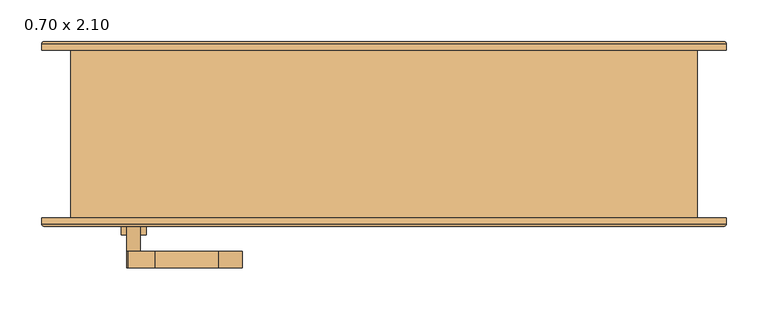
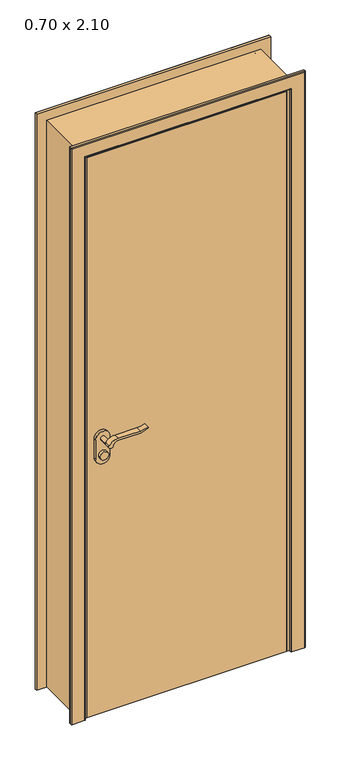
"""IFC4 building model written with IfcOpenShell, lengths in millimetres: door geometry, .CC_ND 300_PORTA SIMPLES DE ABRIR_COM EXTENSÃO : 0.70 x 2.10."""

from ifc_helpers import new_model, si_unit, point, frame, frame_2d, origin, origin_with_axes, place, context, project, spatial, polyline, circle_curve, ellipse_curve, trimmed, segment, composite_curve, outline, extrude, faceted_brep, source, transform, mapped, element, save
from ifc_brep_helpers import plane_surface, cylinder_surface, advanced_brep


def door_0_70_x_2_10_b55f3723(model_context):
    return source(origin(), model_context, "Body", "SolidModel", [
        extrude(outline(composite_curve([segment(trimmed(circle_curve(frame_2d((964.5, -300.0)), 15.0), [point((964.5, -285.0))], [point((964.5, -315.0))], False, "CARTESIAN"), True, "CONTINUOUS"), segment(trimmed(circle_curve(frame_2d((964.5, -300.0)), 15.0), [point((964.5, -315.0))], [point((964.5, -285.0))], False, "CARTESIAN"), True, "CONTINUOUS")], self_intersect=False)), frame((0.0, -120.7, 0.0), z_axis=(0.0, 1.0, 0.0), x_axis=(0.0, 0.0, 1.0)), (0.0, 0.0, 1.0), 10.0),
        extrude(outline(composite_curve([segment(trimmed(circle_curve(frame_2d((964.5, -300.0)), 15.0), [point((964.5, -285.0))], [point((964.5, -315.0))], False, "CARTESIAN"), True, "CONTINUOUS"), segment(trimmed(circle_curve(frame_2d((964.5, -300.0)), 15.0), [point((964.5, -315.0))], [point((964.5, -285.0))], False, "CARTESIAN"), True, "CONTINUOUS")], self_intersect=False)), frame((0.0, -60.7, 0.0), z_axis=(0.0, 1.0, 0.0), x_axis=(0.0, 0.0, 1.0)), (0.0, 0.0, 1.0), 10.0),
        extrude(outline(composite_curve([segment(trimmed(circle_curve(frame_2d((1024.5, -300.0)), 8.0), [point((1029.1523287, -306.5081363))], [point((1024.5, -292.0))], False, "CARTESIAN"), True, "CONTINUOUS"), segment(trimmed(circle_curve(frame_2d((1019.3738613, -274.6138099)), 18.1261387), [point((1024.5, -292.0))], [point((1037.5, -274.6138099))], True, "CARTESIAN"), True, "CONTINUOUS"), segment(polyline([(1037.5, -274.6138099), (1037.5, -198.3564091)]), True, "CONTINUOUS"), segment(trimmed(circle_curve(frame_2d((1096.7709207, -201.9396612)), 59.3791355), [point((1037.5, -198.3564091))], [point((1046.7135558, -170.0))], False, "CARTESIAN"), True, "CONTINUOUS"), segment(polyline([(1046.7135558, -170.0), (1049.5, -170.0)]), True, "CONTINUOUS"), segment(trimmed(circle_curve(frame_2d((1127.7850638, -198.4227909)), 83.2850902), [point((1049.5, -170.0))], [point((1044.5, -198.3564091))], True, "CARTESIAN"), True, "CONTINUOUS"), segment(polyline([(1044.5, -198.3564091), (1044.5, -274.6325667)]), True, "CONTINUOUS"), segment(trimmed(circle_curve(frame_2d((1007.2555521, -276.3324871)), 37.2832219), [point((1044.5, -274.6325667))], [point((1029.1523287, -306.5081363))], False, "CARTESIAN"), True, "CONTINUOUS")], self_intersect=False)), frame((0.0, -160.7, 0.0), z_axis=(0.0, 1.0, 0.0), x_axis=(0.0, 0.0, 1.0)), (0.0, 0.0, 1.0), 20.0),
        extrude(outline(composite_curve([segment(trimmed(circle_curve(frame_2d((1019.3738682, -274.6138122)), 18.1261318), [point((1024.4999903, -292.0))], [point((1037.5, -274.6138122))], True, "CARTESIAN"), True, "CONTINUOUS"), segment(polyline([(1037.5, -274.6138122), (1037.5, -198.3564091)]), True, "CONTINUOUS"), segment(trimmed(circle_curve(frame_2d((1096.7709207, -201.9396612)), 59.3791355), [point((1037.5, -198.3564091))], [point((1046.7135558, -170.0))], False, "CARTESIAN"), True, "CONTINUOUS"), segment(polyline([(1046.7135558, -170.0), (1049.5, -170.0)]), True, "CONTINUOUS"), segment(trimmed(circle_curve(frame_2d((1127.7850638, -198.4227909)), 83.2850902), [point((1049.5, -170.0))], [point((1044.5, -198.3564091))], True, "CARTESIAN"), True, "CONTINUOUS"), segment(polyline([(1044.5, -198.3564091), (1044.5, -274.6325667)]), True, "CONTINUOUS"), segment(trimmed(circle_curve(frame_2d((1007.2555521, -276.3324871)), 37.2832219), [point((1044.5, -274.6325667))], [point((1029.1523287, -306.5081363))], False, "CARTESIAN"), True, "CONTINUOUS"), segment(trimmed(circle_curve(frame_2d((1024.5, -300.0)), 8.0), [point((1029.1523287, -306.5081363))], [point((1024.4999903, -292.0))], False, "CARTESIAN"), True, "CONTINUOUS")], self_intersect=False)), frame((0.0, -30.7, 0.0), z_axis=(0.0, 1.0, 0.0), x_axis=(0.0, 0.0, 1.0)), (0.0, 0.0, 1.0), 20.0),
        extrude(outline(composite_curve([segment(trimmed(circle_curve(frame_2d((1024.5, -300.0)), 8.0), [point((1024.5, -292.0))], [point((1024.5, -308.0))], False, "CARTESIAN"), True, "CONTINUOUS"), segment(trimmed(circle_curve(frame_2d((1024.5, -300.0)), 8.0), [point((1024.5, -308.0))], [point((1024.5, -292.0))], False, "CARTESIAN"), True, "CONTINUOUS")], self_intersect=False)), frame((0.0, -140.7, 0.0), z_axis=(0.0, 1.0, 0.0), x_axis=(0.0, 0.0, 1.0)), (0.0, 0.0, 1.0), 30.0),
        extrude(outline(composite_curve([segment(trimmed(circle_curve(frame_2d((1024.5, -300.0)), 8.0), [point((1024.5, -292.0))], [point((1024.5, -308.0))], False, "CARTESIAN"), True, "CONTINUOUS"), segment(trimmed(circle_curve(frame_2d((1024.5, -300.0)), 8.0), [point((1024.5, -308.0))], [point((1024.5, -292.0))], False, "CARTESIAN"), True, "CONTINUOUS")], self_intersect=False)), frame((0.0, -60.7, 0.0), z_axis=(0.0, 1.0, 0.0), x_axis=(0.0, 0.0, 1.0)), (0.0, 0.0, 1.0), 30.0),
        extrude(outline(composite_curve([segment(trimmed(circle_curve(frame_2d((954.5, -300.0)), 25.0), [point((954.5, -325.0))], [point((954.5, -275.0))], False, "CARTESIAN"), True, "CONTINUOUS"), segment(polyline([(954.5, -275.0), (1024.5, -275.0)]), True, "CONTINUOUS"), segment(trimmed(circle_curve(frame_2d((1024.5, -300.0)), 25.0), [point((1024.5, -275.0))], [point((1024.5, -325.0))], False, "CARTESIAN"), True, "CONTINUOUS"), segment(polyline([(1024.5, -325.0), (954.5, -325.0)]), True, "CONTINUOUS")], self_intersect=False)), frame((0.0, -110.7, 0.0), z_axis=(0.0, 1.0, 0.0), x_axis=(0.0, 0.0, 1.0)), (0.0, 0.0, 1.0), 10.0),
        extrude(outline(composite_curve([segment(trimmed(circle_curve(frame_2d((954.5, -300.0)), 25.0), [point((954.5, -325.0))], [point((954.5, -275.0))], False, "CARTESIAN"), True, "CONTINUOUS"), segment(polyline([(954.5, -275.0), (1024.5, -275.0)]), True, "CONTINUOUS"), segment(trimmed(circle_curve(frame_2d((1024.5, -300.0)), 25.0), [point((1024.5, -275.0))], [point((1024.5, -325.0))], False, "CARTESIAN"), True, "CONTINUOUS"), segment(polyline([(1024.5, -325.0), (954.5, -325.0)]), True, "CONTINUOUS")], self_intersect=False)), frame((0.0, -70.7, 0.0), z_axis=(0.0, 1.0, 0.0), x_axis=(0.0, 0.0, 1.0)), (0.0, 0.0, 1.0), 10.0),
        faceted_brep([(342.0, 100.7, 0.0), (375.0, 100.7, 0.0), (375.0, -100.7, 0.0), (350.0, -100.7, 0.0), (350.0, -70.7, 0.0), (342.0, -70.7, 0.0), (342.0, 100.7, 2067.0), (-342.0, 100.7, 2067.0), (-342.0, 100.7, 0.0), (-375.0, 100.7, 0.0), (-375.0, 100.7, 2100.0), (375.0, 100.7, 2100.0), (375.0, -100.7, 2100.0), (-375.0, -100.7, 2100.0), (-375.0, -100.7, 0.0), (-350.0, -100.7, 0.0), (-350.0, -100.7, 2075.0), (350.0, -100.7, 2075.0), (350.0, -70.7, 2075.0), (-350.0, -70.7, 2075.0), (-350.0, -70.7, 0.0), (-342.0, -70.7, 0.0), (-342.0, -70.7, 2067.0), (342.0, -70.7, 2067.0)], [[[0, 1, 2, 3, 4, 5]], [[1, 0, 6, 7, 8, 9, 10, 11]], [[2, 1, 11, 12]], [[3, 2, 12, 13, 14, 15, 16, 17]], [[4, 3, 17, 18]], [[5, 4, 18, 19, 20, 21, 22, 23]], [[0, 5, 23, 6]], [[7, 22, 21, 8]], [[8, 21, 20, 15, 14, 9]], [[13, 10, 9, 14]], [[19, 16, 15, 20]], [[12, 11, 10, 13]], [[18, 17, 16, 19]], [[6, 23, 22, 7]]]),
        extrude(outline(polyline([(-350.0, -70.7), (350.0, -70.7), (350.0, -100.7), (-350.0, -100.7), (-350.0, -70.7)])), origin_with_axes(), (0.0, 0.0, 1.0), 2075.0),
        advanced_brep(
        [(-410.0, -100.7, 0.0), (-360.0, -100.7, 0.0), (-360.0, -107.7, 0.0), (-363.0, -110.7, 0.0), (-407.0, -110.7, 0.0), (-410.0, -107.7, 0.0), (-410.0, -100.7, 2135.0), (410.0, -100.7, 2135.0), (410.0, -100.7, 0.0), (360.0, -100.7, 0.0), (360.0, -100.7, 2085.0), (-360.0, -100.7, 2085.0), (-360.0, -107.7, 2085.0), (-363.0, -110.7, 2088.0), (363.0, -110.7, 2088.0), (363.0, -110.7, 0.0), (407.0, -110.7, 0.0), (407.0, -110.7, 2132.0), (-407.0, -110.7, 2132.0), (-410.0, -107.7, 2135.0), (410.0, -107.7, 2135.0), (410.0, -107.7, 0.0), (360.0, -107.7, 0.0), (360.0, -107.7, 2085.0)],
        [
            (0, 1),
            (1, 2),
            (2, 3, circle_curve(frame((-363.0, -107.7, 0.0), z_axis=(0.0, 0.0, -1.0), x_axis=(1.0, 0.0, 0.0)), 3.0)),
            (3, 4),
            (4, 5, circle_curve(frame((-407.0, -107.7, 0.0), z_axis=(0.0, 0.0, -1.0), x_axis=(1.0, 0.0, 0.0)), 3.0)),
            (5, 0),
            (0, 6),
            (6, 7),
            (7, 8),
            (8, 9),
            (9, 10),
            (10, 11),
            (11, 1),
            (11, 12),
            (12, 2),
            (12, 13, ellipse_curve(frame((-363.0, -107.7, 2088.0), z_axis=(-0.7071067811865475, 0.0, -0.7071067811865475), x_axis=(0.7071067811865474, 0.0, -0.7071067811865476)), 4.2426407, 3.0)),
            (13, 3),
            (13, 14),
            (14, 15),
            (15, 16),
            (16, 17),
            (17, 18),
            (18, 4),
            (18, 19, ellipse_curve(frame((-407.0, -107.7, 2132.0), z_axis=(-0.7071067811865475, 0.0, -0.7071067811865475), x_axis=(0.7071067811865474, 0.0, -0.7071067811865476)), 4.2426407, 3.0)),
            (19, 5),
            (19, 6),
            (7, 20),
            (20, 21),
            (21, 8),
            (21, 16, circle_curve(frame((407.0, -107.7, 0.0), z_axis=(0.0, 0.0, -1.0), x_axis=(-1.0, 0.0, 0.0)), 3.0)),
            (15, 22, circle_curve(frame((363.0, -107.7, 0.0), z_axis=(0.0, 0.0, -1.0), x_axis=(-1.0, 0.0, 0.0)), 3.0)),
            (22, 9),
            (23, 10),
            (22, 23),
            (14, 23, ellipse_curve(frame((363.0, -107.7, 2088.0), z_axis=(0.7071067811865475, 0.0, -0.7071067811865475), x_axis=(0.7071067811865474, 0.0, 0.7071067811865476)), 4.2426407, 3.0)),
            (20, 17, ellipse_curve(frame((407.0, -107.7, 2132.0), z_axis=(0.7071067811865475, 0.0, -0.7071067811865475), x_axis=(0.7071067811865474, 0.0, 0.7071067811865476)), 4.2426407, 3.0)),
            (23, 12),
            (19, 20),
        ],
        [
            plane_surface(frame((-360.0, -100.7, 0.0), z_axis=(0.0, 0.0, -1.0), x_axis=(0.0, 1.0, 0.0))),
            plane_surface(frame((-410.0, -100.7, 0.0), z_axis=(0.0, 1.0, 0.0), x_axis=(0.0, 0.0, 1.0))),
            plane_surface(frame((-360.0, -100.7, 0.0), z_axis=(1.0, 0.0, 0.0), x_axis=(0.0, 0.0, 1.0))),
            cylinder_surface(frame((-363.0, -107.7, 0.0), z_axis=(0.0, 0.0, -1.0), x_axis=(1.0, 0.0, 0.0)), 3.0),
            plane_surface(frame((-363.0, -110.7, 0.0), z_axis=(0.0, -1.0, 0.0), x_axis=(0.0, 0.0, 1.0))),
            cylinder_surface(frame((-407.0, -107.7, 0.0), z_axis=(0.0, 0.0, -1.0), x_axis=(1.0, 0.0, 0.0)), 3.0),
            plane_surface(frame((-410.0, -107.7, 0.0), z_axis=(-1.0, 0.0, 0.0), x_axis=(0.0, 0.0, 1.0))),
            plane_surface(frame((410.0, -107.7, 2135.0), z_axis=(1.0, 0.0, 0.0), x_axis=(0.0, 0.0, -1.0))),
            plane_surface(frame((360.0, -100.7, 0.0), z_axis=(0.0, 0.0, -1.0), x_axis=(0.0, 1.0, 0.0))),
            plane_surface(frame((360.0, -100.7, 2085.0), z_axis=(-1.0, 0.0, 0.0), x_axis=(0.0, 0.0, -1.0))),
            cylinder_surface(frame((363.0, -107.7, 2085.0), z_axis=(0.0, 0.0, 1.0), x_axis=(-1.0, 0.0, 0.0)), 3.0),
            cylinder_surface(frame((407.0, -107.7, 2085.0), z_axis=(0.0, 0.0, 1.0), x_axis=(-1.0, 0.0, 0.0)), 3.0),
            plane_surface(frame((-360.0, -100.7, 2085.0), z_axis=(0.0, 0.0, -1.0), x_axis=(1.0, 0.0, 0.0))),
            plane_surface(frame((-410.0, -107.7, 2135.0), z_axis=(0.0, 0.0, 1.0), x_axis=(1.0, 0.0, 0.0))),
            cylinder_surface(frame((-360.0, -107.7, 2088.0), z_axis=(-1.0, 0.0, 0.0), x_axis=(0.0, 0.0, -1.0)), 3.0),
            cylinder_surface(frame((-360.0, -107.7, 2132.0), z_axis=(-1.0, 0.0, 0.0), x_axis=(0.0, 0.0, -1.0)), 3.0),
        ],
        [
            (0, [[1, 2, 3, 4, 5, 6]]),
            (1, [[-1, 7, 8, 9, 10, 11, 12, 13]]),
            (2, [[-2, -13, 14, 15]]),
            (3, [[-3, -15, 16, 17]]),
            (4, [[-4, -17, 18, 19, 20, 21, 22, 23]]),
            (5, [[-5, -23, 24, 25]]),
            (6, [[-6, -25, 26, -7]]),
            (7, [[27, 28, 29, -9]]),
            (8, [[-29, 30, -20, 31, 32, -10]]),
            (9, [[33, -11, -32, 34]]),
            (10, [[35, -34, -31, -19]]),
            (11, [[36, -21, -30, -28]]),
            (12, [[-14, -12, -33, 37]]),
            (13, [[-26, 38, -27, -8]]),
            (14, [[-16, -37, -35, -18]]),
            (15, [[-24, -22, -36, -38]]),
        ],
    ),
        advanced_brep(
        [(410.0, 100.7, 0.0), (360.0, 100.7, 0.0), (360.0, 107.7157283, 0.0), (362.9842717, 110.7, 0.0), (407.0342217, 110.7, 0.0), (410.0, 107.7342217, 0.0), (410.0, 100.7, 2135.0), (-410.0, 100.7, 2135.0), (-410.0, 100.7, 0.0), (-360.0, 100.7, 0.0), (-360.0, 100.7, 2085.0), (360.0, 100.7, 2085.0), (360.0, 107.7157283, 2085.0), (362.9842717, 110.7, 2087.9842717), (-362.9842717, 110.7, 2087.9842717), (-362.9842717, 110.7, 0.0), (-407.0342217, 110.7, 0.0), (-407.0342217, 110.7, 2132.0342217), (407.0342217, 110.7, 2132.0342217), (410.0, 107.7342217, 2135.0), (-410.0, 107.7342217, 2135.0), (-410.0, 107.7342217, 0.0), (-360.0, 107.7157283, 0.0), (-360.0, 107.7157283, 2085.0)],
        [
            (0, 1),
            (1, 2),
            (2, 3, circle_curve(frame((362.9842717, 107.7157283, 0.0), z_axis=(0.0, 0.0, -1.0), x_axis=(1.0, 0.0, 0.0)), 2.9842717)),
            (3, 4),
            (4, 5, circle_curve(frame((407.0342217, 107.7342217, 0.0), z_axis=(0.0, 0.0, -1.0), x_axis=(1.0, 0.0, 0.0)), 2.9657783)),
            (5, 0),
            (0, 6),
            (6, 7),
            (7, 8),
            (8, 9),
            (9, 10),
            (10, 11),
            (11, 1),
            (11, 12),
            (12, 2),
            (12, 13, ellipse_curve(frame((362.9842717, 107.7157283, 2087.9842717), z_axis=(0.7071067811865475, 0.0, -0.7071067811865475), x_axis=(-0.7071067811865474, 0.0, -0.7071067811865476)), 4.2203975, 2.9842717)),
            (13, 3),
            (13, 14),
            (14, 15),
            (15, 16),
            (16, 17),
            (17, 18),
            (18, 4),
            (18, 19, ellipse_curve(frame((407.0342217, 107.7342217, 2132.0342217), z_axis=(0.7071067811865475, 0.0, -0.7071067811865475), x_axis=(-0.7071067811865474, 0.0, -0.7071067811865476)), 4.1942438, 2.9657783)),
            (19, 5),
            (19, 6),
            (7, 20),
            (20, 21),
            (21, 8),
            (21, 16, circle_curve(frame((-407.0342217, 107.7342217, 0.0), z_axis=(0.0, 0.0, -1.0), x_axis=(-1.0, 0.0, 0.0)), 2.9657783)),
            (15, 22, circle_curve(frame((-362.9842717, 107.7157283, 0.0), z_axis=(0.0, 0.0, -1.0), x_axis=(-1.0, 0.0, 0.0)), 2.9842717)),
            (22, 9),
            (23, 10),
            (22, 23),
            (14, 23, ellipse_curve(frame((-362.9842717, 107.7157283, 2087.9842717), z_axis=(-0.7071067811865475, 0.0, -0.7071067811865475), x_axis=(-0.7071067811865474, 0.0, 0.7071067811865476)), 4.2203975, 2.9842717)),
            (20, 17, ellipse_curve(frame((-407.0342217, 107.7342217, 2132.0342217), z_axis=(-0.7071067811865475, 0.0, -0.7071067811865475), x_axis=(-0.7071067811865474, 0.0, 0.7071067811865476)), 4.1942438, 2.9657783)),
            (23, 12),
            (19, 20),
        ],
        [
            plane_surface(frame((360.0, 100.7, 0.0), z_axis=(0.0, 0.0, -1.0), x_axis=(0.0, 1.0, 0.0))),
            plane_surface(frame((410.0, 100.7, 0.0), z_axis=(0.0, -1.0, 0.0), x_axis=(0.0, 0.0, 1.0))),
            plane_surface(frame((360.0, 100.7, 0.0), z_axis=(-1.0, 0.0, 0.0), x_axis=(0.0, 0.0, 1.0))),
            cylinder_surface(frame((362.9842717, 107.7157283, 0.0), z_axis=(0.0, 0.0, -1.0), x_axis=(1.0, 0.0, 0.0)), 2.9842717),
            plane_surface(frame((362.9842717, 110.7, 0.0), z_axis=(0.0, 1.0, 0.0), x_axis=(0.0, 0.0, 1.0))),
            cylinder_surface(frame((407.0342217, 107.7342217, 0.0), z_axis=(0.0, 0.0, -1.0), x_axis=(1.0, 0.0, 0.0)), 2.9657783),
            plane_surface(frame((410.0, 107.7342217, 0.0), z_axis=(1.0, 0.0, 0.0), x_axis=(0.0, 0.0, 1.0))),
            plane_surface(frame((-410.0, 107.7342217, 2135.0), z_axis=(-1.0, 0.0, 0.0), x_axis=(0.0, 0.0, -1.0))),
            plane_surface(frame((-360.0, 100.7, 0.0), z_axis=(0.0, 0.0, -1.0), x_axis=(0.0, 1.0, 0.0))),
            plane_surface(frame((-360.0, 100.7, 2085.0), z_axis=(1.0, 0.0, 0.0), x_axis=(0.0, 0.0, -1.0))),
            cylinder_surface(frame((-362.9842717, 107.7157283, 2085.0), z_axis=(0.0, 0.0, 1.0), x_axis=(-1.0, 0.0, 0.0)), 2.9842717),
            cylinder_surface(frame((-407.0342217, 107.7342217, 2085.0), z_axis=(0.0, 0.0, 1.0), x_axis=(-1.0, 0.0, 0.0)), 2.9657783),
            plane_surface(frame((360.0, 100.7, 2085.0), z_axis=(0.0, 0.0, -1.0), x_axis=(-1.0, 0.0, 0.0))),
            plane_surface(frame((410.0, 107.7342217, 2135.0), z_axis=(0.0, 0.0, 1.0), x_axis=(-1.0, 0.0, 0.0))),
            cylinder_surface(frame((360.0, 107.7157283, 2087.9842717), z_axis=(1.0, 0.0, 0.0), x_axis=(0.0, 0.0, 1.0)), 2.9842717),
            cylinder_surface(frame((360.0, 107.7342217, 2132.0342217), z_axis=(1.0, 0.0, 0.0), x_axis=(0.0, 0.0, 1.0)), 2.9657783),
        ],
        [
            (0, [[1, 2, 3, 4, 5, 6]]),
            (1, [[-1, 7, 8, 9, 10, 11, 12, 13]]),
            (2, [[-2, -13, 14, 15]]),
            (3, [[-3, -15, 16, 17]]),
            (4, [[-4, -17, 18, 19, 20, 21, 22, 23]]),
            (5, [[-5, -23, 24, 25]]),
            (6, [[-6, -25, 26, -7]]),
            (7, [[27, 28, 29, -9]]),
            (8, [[-29, 30, -20, 31, 32, -10]]),
            (9, [[33, -11, -32, 34]]),
            (10, [[35, -34, -31, -19]]),
            (11, [[36, -21, -30, -28]]),
            (12, [[-14, -12, -33, 37]]),
            (13, [[-26, 38, -27, -8]]),
            (14, [[-16, -37, -35, -18]]),
            (15, [[-24, -22, -36, -38]]),
        ],
    ),
    ])


if __name__ == "__main__":
    model = new_model("IFC4")
    model_context = context("Model", 3, world=origin())
    ifc_project = project(units=[si_unit("LENGTHUNIT", "METRE", prefix="MILLI")], contexts=[model_context])
    site = spatial("IfcSite", under=ifc_project)
    building = spatial("IfcBuilding", under=site)
    placement = place(None, origin())
    door_0_70_x_2_10_shape = door_0_70_x_2_10_b55f3723(model_context)
    element("IfcDoor", 1, ObjectType=".CC_ND 300_PORTA SIMPLES DE ABRIR_COM EXTENSÃO : 0.70 x 2.10", at=placement, inside=building, context=model_context, shape_type="MappedRepresentation", body=[
        mapped(door_0_70_x_2_10_shape, transform((0.0, 0.0, 0.0), x_axis=(1.0, 0.0, 0.0), y_axis=(0.0, 1.0, 0.0), z_axis=(0.0, 0.0, 1.0))),
    ])
    save(model, "model.ifc")

# Revit data of these elements
# Type ".CC_ND 300_PORTA SIMPLES DE ABRIR_COM EXTENSÃO : 0.70 x 2.10"
#   Type Mark = "155"
#   Analytic Construction = "<None>"
#   Rough Width = 0.75 m
#   Espessura moldura externa = 0.01 m
#   Espessura moldura interna = 0.01 m
#   Largura moldura = 0.05 m
#   Extensão acabamento exterior [instance default] = 0.00 m
#   Extensão acabamento interior [instance default] = 0.00 m
#   Espessura batente = 0.025 m
#   Thickness = 0.03 m
#   Altura batente = 2.085 m
#   Aux Arco [instance default] = 0.70 m
#   Rough Height = 2.125 m
#   Height = 2.10 m
#   Width = 0.70 m
#   Moldura interna [instance default] = yes
#   Moldura externa [instance default] = yes
#   Porta = .MADEIRA COM PINTURA ESMALTE BRANCO ACETINADO
#   Moldura = .MADEIRA COM PINTURA ESMALTE BRANCO ACETINADO
#   Maçaneta = .ALUMÍNIO
#   Batente = .MADEIRA COM PINTURA ESMALTE BRANCO ACETINADO
#   Function = (empty or 0)
#   Wall Closure = (empty or 0)
# Element 1 (IfcDoor, ".CC_ND 300_PORTA SIMPLES DE ABRIR_COM EXTENSÃO : 0.70 x 2.10")
#   Extensão acabamento exterior = 0.0257 m
#   Extensão acabamento interior = 0.0257 m
#   Aux Arco = 0.7257 m
#   Materials on its faces: ".MADEIRA COM PINTURA ESMALTE BRANCO ACETINADO", ".ALUMÍNIO"
# Materials
#   ".MADEIRA COM PINTURA ESMALTE BRANCO ACETINADO": class ".CC_MADEIRAS", colour RGB 240 240 240, transparency 0, Description = "Madeira com pintura esmalte branco acetinado.", Cost = 0
#   ".ALUMÍNIO": class "CC_METAIS", colour RGB 244 244 244, transparency 0, Description = "Material alumínio", Cost = 0
